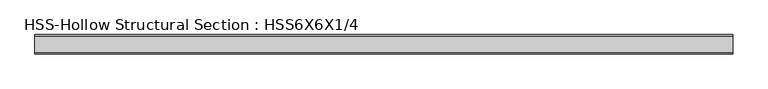
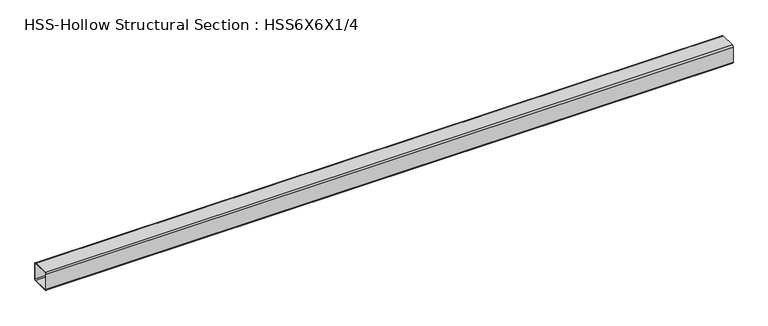
"""IFC4 building model written with IfcOpenShell, lengths in millimetres: beam geometry, HSS-Hollow Structural Section : HSS6X6X1/4."""

from ifc_helpers import new_model, si_unit, point, frame, frame_2d, origin, place, context, project, spatial, polyline, circle_curve, trimmed, segment, composite_curve, outline, extrude, source, transform, mapped, element, save


def hss_hollow_structural_section_hss6x6x1_4_db1f6c85(model_context):
    return source(origin(), model_context, "Body", "SweptSolid", [
        extrude(outline(composite_curve([segment(polyline([(76.2, 64.3636), (76.2, -64.3636)]), True, "CONTINUOUS"), segment(trimmed(circle_curve(frame_2d((64.3636, -64.3636)), 11.8364), [point((76.2, -64.3636))], [point((64.3636, -76.2))], False, "CARTESIAN"), True, "CONTINUOUS"), segment(polyline([(64.3636, -76.2), (-64.3636, -76.2)]), True, "CONTINUOUS"), segment(trimmed(circle_curve(frame_2d((-64.3636, -64.3636)), 11.8364), [point((-64.3636, -76.2))], [point((-76.2, -64.3636))], False, "CARTESIAN"), True, "CONTINUOUS"), segment(polyline([(-76.2, -64.3636), (-76.2, 64.3636)]), True, "CONTINUOUS"), segment(trimmed(circle_curve(frame_2d((-64.3636, 64.3636)), 11.8364), [point((-76.2, 64.3636))], [point((-64.3636, 76.2))], False, "CARTESIAN"), True, "CONTINUOUS"), segment(polyline([(-64.3636, 76.2), (64.3636, 76.2)]), True, "CONTINUOUS"), segment(trimmed(circle_curve(frame_2d((64.3636, 64.3636)), 11.8364), [point((64.3636, 76.2))], [point((76.2, 64.3636))], False, "CARTESIAN"), True, "CONTINUOUS")], self_intersect=False), holes=[composite_curve([segment(trimmed(circle_curve(frame_2d((-64.3636, 64.3636)), 5.9182), [point((-64.3636, 70.2818))], [point((-70.2818, 64.3636))], True, "CARTESIAN"), True, "CONTINUOUS"), segment(polyline([(-70.2818, 64.3636), (-70.2818, -64.3636)]), True, "CONTINUOUS"), segment(trimmed(circle_curve(frame_2d((-64.3636, -64.3636)), 5.9182), [point((-70.2818, -64.3636))], [point((-64.3636, -70.2818))], True, "CARTESIAN"), True, "CONTINUOUS"), segment(polyline([(-64.3636, -70.2818), (64.3636, -70.2818)]), True, "CONTINUOUS"), segment(trimmed(circle_curve(frame_2d((64.3636, -64.3636)), 5.9182), [point((64.3636, -70.2818))], [point((70.2818, -64.3636))], True, "CARTESIAN"), True, "CONTINUOUS"), segment(polyline([(70.2818, -64.3636), (70.2818, 64.3636)]), True, "CONTINUOUS"), segment(trimmed(circle_curve(frame_2d((64.3636, 64.3636)), 5.9182), [point((70.2818, 64.3636))], [point((64.3636, 70.2818))], True, "CARTESIAN"), True, "CONTINUOUS"), segment(polyline([(64.3636, 70.2818), (-64.3636, 70.2818)]), True, "CONTINUOUS")], self_intersect=False)]), frame((-2751.9238693, 0.0, 0.0), z_axis=(1.0, 0.0, 0.0), x_axis=(0.0, 1.0, 0.0)), (0.0, 0.0, 1.0), 5507.8238693),
    ])


if __name__ == "__main__":
    model = new_model("IFC4")
    model_context = context("Model", 3, world=origin())
    ifc_project = project(units=[si_unit("LENGTHUNIT", "METRE", prefix="MILLI")], contexts=[model_context])
    site = spatial("IfcSite", under=ifc_project)
    building = spatial("IfcBuilding", under=site)
    placement = place(None, origin())
    hss_hollow_structural_section_hss6x6x1_4_shape = hss_hollow_structural_section_hss6x6x1_4_db1f6c85(model_context)
    element("IfcBeam", 1, ObjectType="HSS-Hollow Structural Section : HSS6X6X1/4", at=placement, inside=building, context=model_context, shape_type="MappedRepresentation", body=[
        mapped(hss_hollow_structural_section_hss6x6x1_4_shape, transform((0.0, 0.0, 0.0), x_axis=(1.0, 0.0, 0.0), y_axis=(0.0, 1.0, 0.0), z_axis=(0.0, 0.0, 1.0))),
    ])
    save(model, "model.ifc")

# Revit data of these elements
# Type "HSS-Hollow Structural Section : HSS6X6X1/4"
#   Assembly Code = "B10"
#   Shape = "Square"
#   W = 19
#   Ht = 0' - 6"
#   Length [instance default] = 5' - 0"
#   b = 0' - 6"
#   kr = 0' - 0.466"
#   t = 0' - 0.233"
#   A = 0.0363889 SF
#   Structural Material [instance default] = Steel ASTM A500, Grade B, Rectangular and Square
# Element 1 (IfcBeam, "HSS-Hollow Structural Section : HSS6X6X1/4")
#   Materials on its faces: "Steel ASTM A500, Grade B, Rectangular and Square"
# Materials
#   "Steel ASTM A500, Grade B, Rectangular and Square": class "Metal", colour RGB 199 199 199, transparency 0, Description = "Carbon steel", Cost = 0
